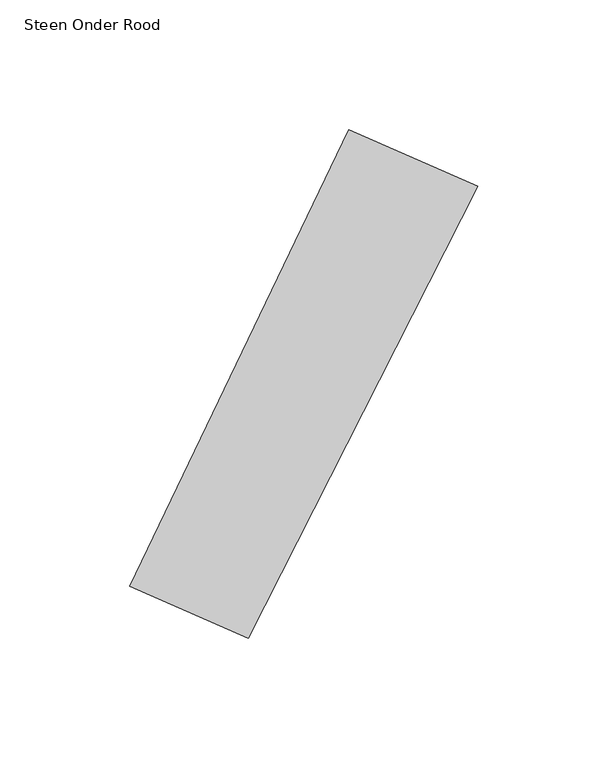
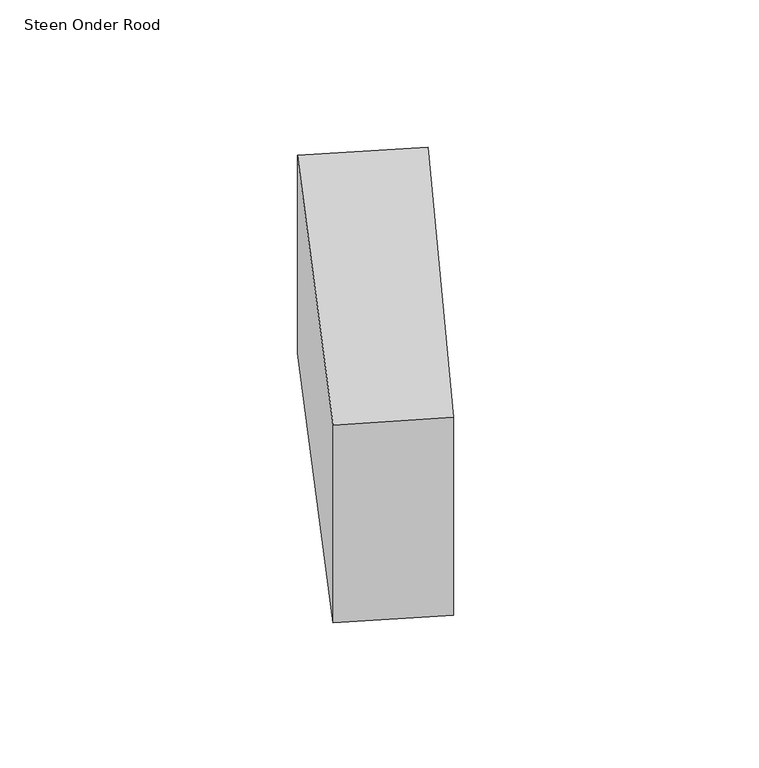
"""IFC4 building model written with IfcOpenShell, lengths in millimetres: proxy geometry, 00_GMA_steen_versie_4 : Steen Onder Rood."""

import ifcopenshell
import ifcopenshell.guid

model = None  # the IFC model being written
_history = None  # IfcOwnerHistory: only IFC2X3 demands one
_inside = {}  # id of a spatial element -> (the spatial element, [elements in it])
_under = {}  # id of a project, library or spatial element -> (it, [spatial elements below it])
_declared = {}  # id of a project -> (the project, [libraries it declares])
_typed = {}  # id of a type object -> (the type object, [elements of that type])
_made_of = {}  # id of a material, layer set ... -> (it, [elements and type objects made of it])


def new_model(schema):
    """Start an empty IFC model of exactly this schema.

    Asked for "IFC4X3", IfcOpenShell would pick the latest addendum, in which some entities
    have other attributes; the version numbers below select the first issue.
    IFC2X3 requires an IfcOwnerHistory on every rooted entity: one is made here for all.
    """
    global model, _history
    if schema == "IFC4X3":
        model = ifcopenshell.file(schema_version=(4, 3, 0, 0))
    else:
        model = ifcopenshell.file(schema=schema)
    _inside.clear()
    _under.clear()
    _declared.clear()
    _typed.clear()
    _made_of.clear()
    _history = None
    if model.schema == "IFC2X3":
        org = make("IfcOrganization", Name="unknown")
        user = make(
            "IfcPersonAndOrganization",
            ThePerson=make("IfcPerson", FamilyName="unknown"),
            TheOrganization=org,
        )
        app = make(
            "IfcApplication",
            ApplicationDeveloper=org,
            Version="unknown",
            ApplicationFullName="unknown",
            ApplicationIdentifier="unknown",
        )
        _history = make(
            "IfcOwnerHistory",
            OwningUser=user,
            OwningApplication=app,
            ChangeAction="ADDED",
            CreationDate=0,
        )
    return model


def make(cls, **values):
    """One entity of the class cls with the attributes given. An attribute that is None is left unset."""
    return model.create_entity(
        cls, **{name: value for name, value in values.items() if value is not None}
    )


def rooted(cls, **values):
    """An entity with a GlobalId (a new one), such as an element, a storey or a relation."""
    return make(cls, GlobalId=ifcopenshell.guid.new(), OwnerHistory=_history, **values)


def si_unit(unit_type, name, prefix=None):
    """IfcSIUnit, for example si_unit("LENGTHUNIT", "METRE", prefix="MILLI")."""
    return make("IfcSIUnit", UnitType=unit_type, Prefix=prefix, Name=name)


def assignment(units):
    """IfcUnitAssignment: the units of a project."""
    return None if units is None else make("IfcUnitAssignment", Units=units)


def point(xyz):
    """IfcCartesianPoint."""
    return None if xyz is None else make("IfcCartesianPoint", Coordinates=xyz)


def direction(xyz):
    """IfcDirection."""
    return None if xyz is None else make("IfcDirection", DirectionRatios=xyz)


def frame(location, z_axis=None, x_axis=None):
    """IfcAxis2Placement3D, a coordinate frame: its origin and axes. An axis left out is left unset."""
    return make(
        "IfcAxis2Placement3D",
        Location=point(location),
        Axis=direction(z_axis),
        RefDirection=direction(x_axis),
    )


def origin():
    """The frame at (0, 0, 0) with its axes left unset."""
    return frame((0.0, 0.0, 0.0))


def origin_with_axes():
    """The frame at (0, 0, 0) with the z axis (0, 0, 1) and the x axis (1, 0, 0) written out."""
    return frame((0.0, 0.0, 0.0), z_axis=(0.0, 0.0, 1.0), x_axis=(1.0, 0.0, 0.0))


def place(relative_to, where):
    """IfcLocalPlacement: puts the frame where relative to a parent placement (None: the world)."""
    return make(
        "IfcLocalPlacement", PlacementRelTo=relative_to, RelativePlacement=where
    )


def context(
    kind, dimensions, precision=None, world=None, true_north=None, identifier=None
):
    """IfcGeometricRepresentationContext, for example the 3D "Model" context."""
    return make(
        "IfcGeometricRepresentationContext",
        ContextIdentifier=identifier,
        ContextType=kind,
        CoordinateSpaceDimension=dimensions,
        Precision=precision,
        WorldCoordinateSystem=world,
        TrueNorth=true_north,
    )


def project(units=None, contexts=None):
    """IfcProject with its units and contexts."""
    return rooted(
        "IfcProject",
        Name="project",
        RepresentationContexts=contexts,
        UnitsInContext=assignment(units),
    )


def spatial(cls, under=None, at=None, **own):
    """A site, building, storey or space (cls), placed at a placement, below another one or the project."""
    s = rooted(cls, ObjectPlacement=at, **own)
    if under is not None:
        _under.setdefault(under.id(), (under, []))[1].append(s)
    return s


def polyline(points):
    """IfcPolyline through the points."""
    return make("IfcPolyline", Points=[point(p) for p in points])


def outline(outer, holes=None, kind="AREA"):
    """IfcArbitraryClosedProfileDef: a profile drawn as a closed curve; with holes, ...WithVoids."""
    if holes is None:
        return make("IfcArbitraryClosedProfileDef", ProfileType=kind, OuterCurve=outer)
    return make(
        "IfcArbitraryProfileDefWithVoids",
        ProfileType=kind,
        OuterCurve=outer,
        InnerCurves=holes,
    )


def extrude(swept, where, along, depth):
    """IfcExtrudedAreaSolid: the profile swept, set in the frame where, extruded along a direction by depth."""
    return make(
        "IfcExtrudedAreaSolid",
        SweptArea=swept,
        Position=where,
        ExtrudedDirection=direction(along),
        Depth=depth,
    )


def shape(context_of_items, identifier, shape_type, items):
    """IfcShapeRepresentation: the items that make up one representation, for example the "Body"."""
    return make(
        "IfcShapeRepresentation",
        ContextOfItems=context_of_items,
        RepresentationIdentifier=identifier,
        RepresentationType=shape_type,
        Items=items,
    )


def source(mapping_origin, context_of_items, identifier, shape_type, items):
    """IfcRepresentationMap: a shape defined once, which mapped items show again and again."""
    return make(
        "IfcRepresentationMap",
        MappingOrigin=mapping_origin,
        MappedRepresentation=shape(context_of_items, identifier, shape_type, items),
    )


def transform(
    local_origin,
    x_axis=None,
    y_axis=None,
    z_axis=None,
    scale=None,
    scale2=None,
    scale3=None,
    uniform=True,
):
    """IfcCartesianTransformationOperator3D, or its non-uniform kind. x_axis, y_axis, z_axis: its Axis1, 2, 3."""
    if uniform:
        return make(
            "IfcCartesianTransformationOperator3D",
            Axis1=direction(x_axis),
            Axis2=direction(y_axis),
            LocalOrigin=point(local_origin),
            Scale=scale,
            Axis3=direction(z_axis),
        )
    return make(
        "IfcCartesianTransformationOperator3DnonUniform",
        Axis1=direction(x_axis),
        Axis2=direction(y_axis),
        LocalOrigin=point(local_origin),
        Scale=scale,
        Axis3=direction(z_axis),
        Scale2=scale2,
        Scale3=scale3,
    )


def mapped(mapping_source, mapping_target):
    """IfcMappedItem: shows the shape of a source again, moved by a transform."""
    return make(
        "IfcMappedItem", MappingSource=mapping_source, MappingTarget=mapping_target
    )


def made_of(thing, what):
    """Note that an element or type object is made of a material, layer set ...; save() writes the relation."""
    if what is not None:
        _made_of.setdefault(what.id(), (what, []))[1].append(thing)
    return thing


def element(
    cls,
    number,
    at=None,
    inside=None,
    cuts=None,
    type_object=None,
    material=None,
    context=None,
    identifier="Body",
    shape_type=None,
    held_by="IfcProductDefinitionShape",
    body=None,
    shapes=None,
    **own,
):
    """One element of the class cls, such as IfcWall. Its Tag is "e" and its number.

    at: its placement. inside: the storey or other place that contains it. cuts: it is an
    opening in that element (IfcRelVoidsElement). A single representation is given by context,
    identifier, shape_type and body (its items); several are given by shapes. held_by: the class
    of the entity that holds the representations. save() writes the other relations.
    """
    e = rooted(cls, Tag="e%d" % number, ObjectPlacement=at, **own)
    if body is not None:
        shapes = [shape(context, identifier, shape_type, body)]
    if shapes is not None:
        e.Representation = make(held_by, Representations=shapes)
    if inside is not None:
        _inside.setdefault(inside.id(), (inside, []))[1].append(e)
    if cuts is not None:
        rooted(
            "IfcRelVoidsElement", RelatingBuildingElement=cuts, RelatedOpeningElement=e
        )
    if type_object is not None:
        _typed.setdefault(type_object.id(), (type_object, []))[1].append(e)
    return made_of(e, material)


def aggregate(whole, parts):
    """IfcRelAggregates: a whole, such as a stair, and the parts it consists of."""
    return rooted("IfcRelAggregates", RelatingObject=whole, RelatedObjects=parts)


def save(model, path):
    """Write the relations noted so far, then the file.

    IfcRelAggregates (storeys below a building ...), IfcRelContainedInSpatialStructure (elements
    in a storey), IfcRelDefinesByType, IfcRelAssociatesMaterial and IfcRelDeclares: one each for
    every whole, place, type object, material and project.
    """
    for whole, parts in _under.values():
        aggregate(whole, parts)
    for where, things in _inside.values():
        rooted(
            "IfcRelContainedInSpatialStructure",
            RelatedElements=things,
            RelatingStructure=where,
        )
    for kind, things in _typed.values():
        rooted("IfcRelDefinesByType", RelatedObjects=things, RelatingType=kind)
    for what, things in _made_of.values():
        rooted("IfcRelAssociatesMaterial", RelatedObjects=things, RelatingMaterial=what)
    for by, libraries in _declared.values():
        rooted("IfcRelDeclares", RelatingContext=by, RelatedDefinitions=libraries)
    model.write(path)


def steen_onder_rood_091d811c(model_context):
    return source(origin(), model_context, "Body", "SweptSolid", [
        extrude(outline(polyline([(144.0475782, 155.4562138), (55.6410388, -18.697475), (9.8698839, 1.4271711), (94.3076096, 177.3213249), (144.0475782, 155.4562138)])), origin_with_axes(), (0.0, 0.0, 1.0), 100.0),
    ])


if __name__ == "__main__":
    model = new_model("IFC4")
    model_context = context("Model", 3, world=origin())
    ifc_project = project(units=[si_unit("LENGTHUNIT", "METRE", prefix="MILLI")], contexts=[model_context])
    site = spatial("IfcSite", under=ifc_project)
    building = spatial("IfcBuilding", under=site)
    placement = place(None, origin())
    steen_onder_rood_shape = steen_onder_rood_091d811c(model_context)
    element("IfcBuildingElementProxy", 1, Name="00_GMA_steen_versie_4 : Steen Onder Rood", ObjectType="00_GMA_steen_versie_4 : Steen Onder Rood", at=placement, inside=building, context=model_context, shape_type="MappedRepresentation", body=[
        mapped(steen_onder_rood_shape, transform((0.0, 0.0, 0.0), x_axis=(1.0, 0.0, 0.0), y_axis=(0.0, 1.0, 0.0), z_axis=(0.0, 0.0, 1.0))),
    ])
    save(model, "model.ifc")

# Revit data of these elements
# Type "00_GMA_steen_versie_4 : Steen Onder Rood"
#   StootVoegHalfBoven [instance default] = 5 mm
#   StootVoegHalf [instance default] = 5 mm
#   StootVoegBreedteOnder = 10 mm
#   StootVoegBreedteBoven = 10 mm
#   Steendikte = 100 mm
#   LintVoegOnderHalf = 0 mm
#   LintVoegOnder = 0 mm
#   LintVoegBovenHalf = 5 mm
#   LintVoegBoven = 10 mm
#   materiaal = 21_steen_rood
#   MateriaalVoeg = none
#   Default Elevation = 0
# Element 1 (IfcBuildingElementProxy, "00_GMA_steen_versie_4 : Steen Onder Rood")
#   Materials on its faces: "21_steen_rood"
# Materials
#   "21_steen_rood": class "Unassigned", colour RGB 213 111 43, transparency 0, Cost = 0
